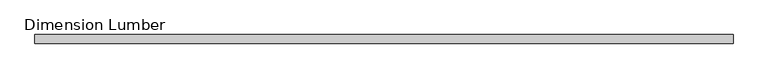
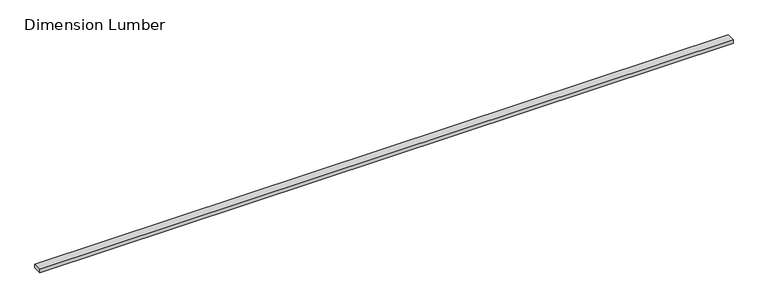
"""IFC4 building model written with IfcOpenShell, lengths in millimetres: beam geometry, Dimension Lumber : Top Supporting Lumbers."""

from ifc_helpers import new_model, si_unit, frame, origin, place, context, project, spatial, polyline, outline, extrude, source, transform, mapped, element, save


def dimension_lumber_a36e28ec(model_context):
    return source(origin(), model_context, "Body", "SweptSolid", [
        extrude(outline(polyline([(3639.34375, 44.45), (3639.34375, -44.45), (-3550.44375, -44.45), (-3550.44375, 44.45), (3639.34375, 44.45)])), frame((0.0, 0.0, -19.05), z_axis=(0.0, 0.0, 1.0), x_axis=(1.0, 0.0, 0.0)), (0.0, 0.0, 1.0), 38.1),
    ])


if __name__ == "__main__":
    model = new_model("IFC4")
    model_context = context("Model", 3, world=origin())
    ifc_project = project(units=[si_unit("LENGTHUNIT", "METRE", prefix="MILLI")], contexts=[model_context])
    site = spatial("IfcSite", under=ifc_project)
    building = spatial("IfcBuilding", under=site)
    placement = place(None, origin())
    dimension_lumber_shape = dimension_lumber_a36e28ec(model_context)
    element("IfcBeam", 1, ObjectType="Dimension Lumber : Top Supporting Lumbers", at=placement, inside=building, context=model_context, shape_type="MappedRepresentation", body=[
        mapped(dimension_lumber_shape, transform((0.0, 0.0, 0.0), x_axis=(1.0, 0.0, 0.0), y_axis=(0.0, 1.0, 0.0), z_axis=(0.0, 0.0, 1.0))),
    ])
    save(model, "model.ifc")

# Revit data of these elements
# Type "Dimension Lumber : Top Supporting Lumbers"
#   Assembly Code = "B10"
#   A = 0.0364583 SF
#   Length [instance default] = 5' - 0"
#   b = 0' - 3 1/2"
#   d = 0' - 1 1/2"
#   Structural Material [instance default] = Softwood, Lumber
# Element 1 (IfcBeam, "Dimension Lumber : Top Supporting Lumbers")
#   Structural Material = Douglas Fir #2
#   Materials on its faces: "Douglas Fir #2"
# Materials
#   "Softwood, Lumber": class "Wood", colour RGB 223 192 134, transparency 0, Description = "Pinus Echinata", Cost = 0
#   "Douglas Fir #2": class "Wood", colour RGB 223 192 134, transparency 0, Description = "Pinus Echinata", Cost = 0
